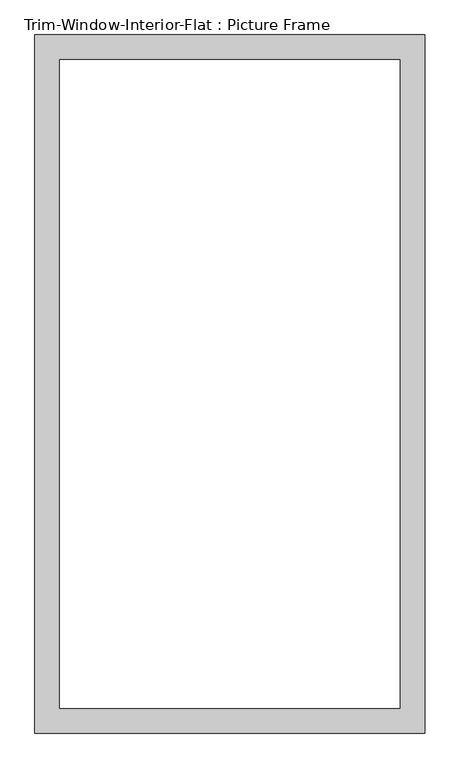
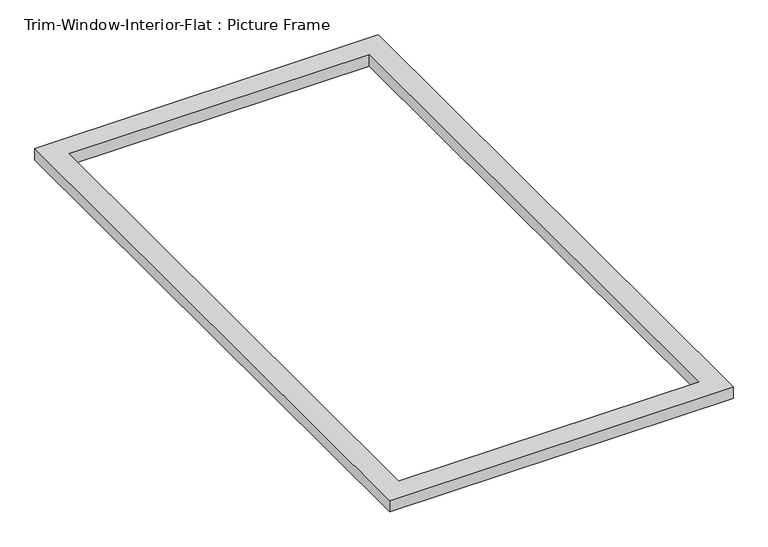
"""IFC4 building model written with IfcOpenShell, lengths in millimetres: proxy geometry, Trim-Window-Interior-Flat : Picture Frame."""

import ifcopenshell
import ifcopenshell.guid

model = None  # the IFC model being written
_history = None  # IfcOwnerHistory: only IFC2X3 demands one
_inside = {}  # id of a spatial element -> (the spatial element, [elements in it])
_under = {}  # id of a project, library or spatial element -> (it, [spatial elements below it])
_declared = {}  # id of a project -> (the project, [libraries it declares])
_typed = {}  # id of a type object -> (the type object, [elements of that type])
_made_of = {}  # id of a material, layer set ... -> (it, [elements and type objects made of it])


def new_model(schema):
    """Start an empty IFC model of exactly this schema.

    Asked for "IFC4X3", IfcOpenShell would pick the latest addendum, in which some entities
    have other attributes; the version numbers below select the first issue.
    IFC2X3 requires an IfcOwnerHistory on every rooted entity: one is made here for all.
    """
    global model, _history
    if schema == "IFC4X3":
        model = ifcopenshell.file(schema_version=(4, 3, 0, 0))
    else:
        model = ifcopenshell.file(schema=schema)
    _inside.clear()
    _under.clear()
    _declared.clear()
    _typed.clear()
    _made_of.clear()
    _history = None
    if model.schema == "IFC2X3":
        org = make("IfcOrganization", Name="unknown")
        user = make(
            "IfcPersonAndOrganization",
            ThePerson=make("IfcPerson", FamilyName="unknown"),
            TheOrganization=org,
        )
        app = make(
            "IfcApplication",
            ApplicationDeveloper=org,
            Version="unknown",
            ApplicationFullName="unknown",
            ApplicationIdentifier="unknown",
        )
        _history = make(
            "IfcOwnerHistory",
            OwningUser=user,
            OwningApplication=app,
            ChangeAction="ADDED",
            CreationDate=0,
        )
    return model


def make(cls, **values):
    """One entity of the class cls with the attributes given. An attribute that is None is left unset."""
    return model.create_entity(
        cls, **{name: value for name, value in values.items() if value is not None}
    )


def rooted(cls, **values):
    """An entity with a GlobalId (a new one), such as an element, a storey or a relation."""
    return make(cls, GlobalId=ifcopenshell.guid.new(), OwnerHistory=_history, **values)


def si_unit(unit_type, name, prefix=None):
    """IfcSIUnit, for example si_unit("LENGTHUNIT", "METRE", prefix="MILLI")."""
    return make("IfcSIUnit", UnitType=unit_type, Prefix=prefix, Name=name)


def assignment(units):
    """IfcUnitAssignment: the units of a project."""
    return None if units is None else make("IfcUnitAssignment", Units=units)


def point(xyz):
    """IfcCartesianPoint."""
    return None if xyz is None else make("IfcCartesianPoint", Coordinates=xyz)


def direction(xyz):
    """IfcDirection."""
    return None if xyz is None else make("IfcDirection", DirectionRatios=xyz)


def frame(location, z_axis=None, x_axis=None):
    """IfcAxis2Placement3D, a coordinate frame: its origin and axes. An axis left out is left unset."""
    return make(
        "IfcAxis2Placement3D",
        Location=point(location),
        Axis=direction(z_axis),
        RefDirection=direction(x_axis),
    )


def origin():
    """The frame at (0, 0, 0) with its axes left unset."""
    return frame((0.0, 0.0, 0.0))


def origin_with_axes():
    """The frame at (0, 0, 0) with the z axis (0, 0, 1) and the x axis (1, 0, 0) written out."""
    return frame((0.0, 0.0, 0.0), z_axis=(0.0, 0.0, 1.0), x_axis=(1.0, 0.0, 0.0))


def place(relative_to, where):
    """IfcLocalPlacement: puts the frame where relative to a parent placement (None: the world)."""
    return make(
        "IfcLocalPlacement", PlacementRelTo=relative_to, RelativePlacement=where
    )


def context(
    kind, dimensions, precision=None, world=None, true_north=None, identifier=None
):
    """IfcGeometricRepresentationContext, for example the 3D "Model" context."""
    return make(
        "IfcGeometricRepresentationContext",
        ContextIdentifier=identifier,
        ContextType=kind,
        CoordinateSpaceDimension=dimensions,
        Precision=precision,
        WorldCoordinateSystem=world,
        TrueNorth=true_north,
    )


def project(units=None, contexts=None):
    """IfcProject with its units and contexts."""
    return rooted(
        "IfcProject",
        Name="project",
        RepresentationContexts=contexts,
        UnitsInContext=assignment(units),
    )


def spatial(cls, under=None, at=None, **own):
    """A site, building, storey or space (cls), placed at a placement, below another one or the project."""
    s = rooted(cls, ObjectPlacement=at, **own)
    if under is not None:
        _under.setdefault(under.id(), (under, []))[1].append(s)
    return s


def polyline(points):
    """IfcPolyline through the points."""
    return make("IfcPolyline", Points=[point(p) for p in points])


def outline(outer, holes=None, kind="AREA"):
    """IfcArbitraryClosedProfileDef: a profile drawn as a closed curve; with holes, ...WithVoids."""
    if holes is None:
        return make("IfcArbitraryClosedProfileDef", ProfileType=kind, OuterCurve=outer)
    return make(
        "IfcArbitraryProfileDefWithVoids",
        ProfileType=kind,
        OuterCurve=outer,
        InnerCurves=holes,
    )


def extrude(swept, where, along, depth):
    """IfcExtrudedAreaSolid: the profile swept, set in the frame where, extruded along a direction by depth."""
    return make(
        "IfcExtrudedAreaSolid",
        SweptArea=swept,
        Position=where,
        ExtrudedDirection=direction(along),
        Depth=depth,
    )


def shape(context_of_items, identifier, shape_type, items):
    """IfcShapeRepresentation: the items that make up one representation, for example the "Body"."""
    return make(
        "IfcShapeRepresentation",
        ContextOfItems=context_of_items,
        RepresentationIdentifier=identifier,
        RepresentationType=shape_type,
        Items=items,
    )


def source(mapping_origin, context_of_items, identifier, shape_type, items):
    """IfcRepresentationMap: a shape defined once, which mapped items show again and again."""
    return make(
        "IfcRepresentationMap",
        MappingOrigin=mapping_origin,
        MappedRepresentation=shape(context_of_items, identifier, shape_type, items),
    )


def transform(
    local_origin,
    x_axis=None,
    y_axis=None,
    z_axis=None,
    scale=None,
    scale2=None,
    scale3=None,
    uniform=True,
):
    """IfcCartesianTransformationOperator3D, or its non-uniform kind. x_axis, y_axis, z_axis: its Axis1, 2, 3."""
    if uniform:
        return make(
            "IfcCartesianTransformationOperator3D",
            Axis1=direction(x_axis),
            Axis2=direction(y_axis),
            LocalOrigin=point(local_origin),
            Scale=scale,
            Axis3=direction(z_axis),
        )
    return make(
        "IfcCartesianTransformationOperator3DnonUniform",
        Axis1=direction(x_axis),
        Axis2=direction(y_axis),
        LocalOrigin=point(local_origin),
        Scale=scale,
        Axis3=direction(z_axis),
        Scale2=scale2,
        Scale3=scale3,
    )


def mapped(mapping_source, mapping_target):
    """IfcMappedItem: shows the shape of a source again, moved by a transform."""
    return make(
        "IfcMappedItem", MappingSource=mapping_source, MappingTarget=mapping_target
    )


def made_of(thing, what):
    """Note that an element or type object is made of a material, layer set ...; save() writes the relation."""
    if what is not None:
        _made_of.setdefault(what.id(), (what, []))[1].append(thing)
    return thing


def element(
    cls,
    number,
    at=None,
    inside=None,
    cuts=None,
    type_object=None,
    material=None,
    context=None,
    identifier="Body",
    shape_type=None,
    held_by="IfcProductDefinitionShape",
    body=None,
    shapes=None,
    **own,
):
    """One element of the class cls, such as IfcWall. Its Tag is "e" and its number.

    at: its placement. inside: the storey or other place that contains it. cuts: it is an
    opening in that element (IfcRelVoidsElement). A single representation is given by context,
    identifier, shape_type and body (its items); several are given by shapes. held_by: the class
    of the entity that holds the representations. save() writes the other relations.
    """
    e = rooted(cls, Tag="e%d" % number, ObjectPlacement=at, **own)
    if body is not None:
        shapes = [shape(context, identifier, shape_type, body)]
    if shapes is not None:
        e.Representation = make(held_by, Representations=shapes)
    if inside is not None:
        _inside.setdefault(inside.id(), (inside, []))[1].append(e)
    if cuts is not None:
        rooted(
            "IfcRelVoidsElement", RelatingBuildingElement=cuts, RelatedOpeningElement=e
        )
    if type_object is not None:
        _typed.setdefault(type_object.id(), (type_object, []))[1].append(e)
    return made_of(e, material)


def aggregate(whole, parts):
    """IfcRelAggregates: a whole, such as a stair, and the parts it consists of."""
    return rooted("IfcRelAggregates", RelatingObject=whole, RelatedObjects=parts)


def save(model, path):
    """Write the relations noted so far, then the file.

    IfcRelAggregates (storeys below a building ...), IfcRelContainedInSpatialStructure (elements
    in a storey), IfcRelDefinesByType, IfcRelAssociatesMaterial and IfcRelDeclares: one each for
    every whole, place, type object, material and project.
    """
    for whole, parts in _under.values():
        aggregate(whole, parts)
    for where, things in _inside.values():
        rooted(
            "IfcRelContainedInSpatialStructure",
            RelatedElements=things,
            RelatingStructure=where,
        )
    for kind, things in _typed.values():
        rooted("IfcRelDefinesByType", RelatedObjects=things, RelatingType=kind)
    for what, things in _made_of.values():
        rooted("IfcRelAssociatesMaterial", RelatedObjects=things, RelatingMaterial=what)
    for by, libraries in _declared.values():
        rooted("IfcRelDeclares", RelatingContext=by, RelatedDefinitions=libraries)
    model.write(path)


def trim_window_interior_flat_picture_frame_5b381bd7(model_context):
    return source(origin(), model_context, "Body", "SweptSolid", [
        extrude(outline(polyline([(450.85, 44.45), (450.85, -1568.45), (-450.85, -1568.45), (-450.85, 44.45), (450.85, 44.45)]), holes=[polyline([(393.7, -12.7), (-393.7, -12.7), (-393.7, -1511.3), (393.7, -1511.3), (393.7, -12.7)])]), origin_with_axes(), (0.0, 0.0, 1.0), 31.75),
    ])


if __name__ == "__main__":
    model = new_model("IFC4")
    model_context = context("Model", 3, world=origin())
    ifc_project = project(units=[si_unit("LENGTHUNIT", "METRE", prefix="MILLI")], contexts=[model_context])
    site = spatial("IfcSite", under=ifc_project)
    building = spatial("IfcBuilding", under=site)
    placement = place(None, origin())
    trim_window_interior_flat_picture_frame_shape = trim_window_interior_flat_picture_frame_5b381bd7(model_context)
    element("IfcBuildingElementProxy", 1, Name="Trim-Window-Interior-Flat : Picture Frame", ObjectType="Trim-Window-Interior-Flat : Picture Frame", at=placement, inside=building, context=model_context, shape_type="MappedRepresentation", body=[
        mapped(trim_window_interior_flat_picture_frame_shape, transform((0.0, 0.0, 0.0), x_axis=(1.0, 0.0, 0.0), y_axis=(0.0, 1.0, 0.0), z_axis=(0.0, 0.0, 1.0))),
    ])
    save(model, "model.ifc")

# Revit data of these elements
# Type "Trim-Window-Interior-Flat : Picture Frame"
#   Trim Thickness_Picture Frame = 0' - 1 1/4"
#   Trim Width = 0' - 2 1/4"
#   Trim Thickness_with Sill = 0' - 0 3/4"
#   Sill Thickness = 0' - 1 1/4"
#   Opening Width [instance default] = 2' - 0"
#   Opening Height [instance default] = 3' - 0"
#   Default Elevation = 4' - 0"
#   Sill = no
#   Picture Frame = yes
#   Trim Material [instance default] = none
# Element 1 (IfcBuildingElementProxy, "Trim-Window-Interior-Flat : Picture Frame")
#   Opening Width = 2' - 8"
#   Opening Height = 5' - 0"
#   Trim Material = Wood - Stained
#   Materials on its faces: "Wood - Stained"
# Materials
#   "Wood - Stained": class "Wood", colour RGB 224 178 126, transparency 0, Cost = 0
